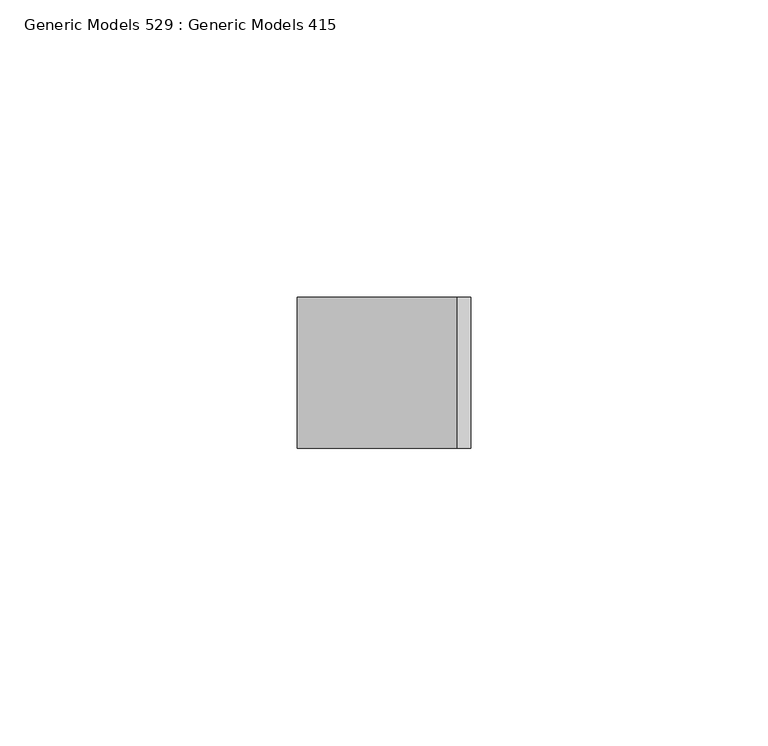
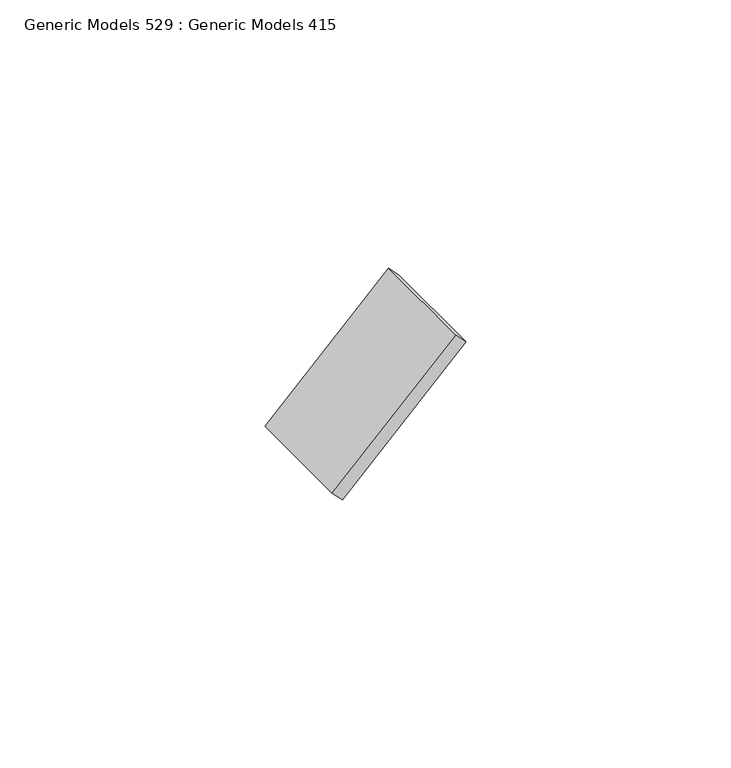
"""IFC4 building model written with IfcOpenShell, lengths in millimetres: proxy geometry, Generic Models 529 : Generic Models 415."""

from ifc_helpers import new_model, si_unit, frame, origin, place, context, project, spatial, polyline, outline, extrude, source, transform, mapped, element, save


def generic_models_529_generic_models_415_c3eaaae7(model_context):
    return source(origin(), model_context, "Body", "SweptSolid", [
        extrude(outline(polyline([(0.0, -3.175), (0.0, 0.0), (25.4, 0.0), (25.4, -3.175), (0.0, -3.175)])), frame((7848.0411784, 4501.3863946, 125384.8849742), z_axis=(0.7071067811867181, 0.0, 0.707106781186377), x_axis=(0.0, -1.0, 0.0)), (0.0, 0.0, 1.0), 38.1),
    ])


if __name__ == "__main__":
    model = new_model("IFC4")
    model_context = context("Model", 3, world=origin())
    ifc_project = project(units=[si_unit("LENGTHUNIT", "METRE", prefix="MILLI")], contexts=[model_context])
    site = spatial("IfcSite", under=ifc_project)
    building = spatial("IfcBuilding", under=site)
    placement = place(None, origin())
    generic_models_529_generic_models_415_shape = generic_models_529_generic_models_415_c3eaaae7(model_context)
    element("IfcBuildingElementProxy", 1, Name="Generic Models 529 : Generic Models 415", ObjectType="Generic Models 529 : Generic Models 415", at=placement, inside=building, context=model_context, shape_type="MappedRepresentation", body=[
        mapped(generic_models_529_generic_models_415_shape, transform((0.0, 0.0, 0.0), x_axis=(1.0, 0.0, 0.0), y_axis=(0.0, 1.0, 0.0), z_axis=(0.0, 0.0, 1.0))),
    ])
    save(model, "model.ifc")

# Revit data of these elements
# Element 1 (IfcBuildingElementProxy, "Generic Models 529 : Generic Models 415")
#   Materials on its faces: "_WELDED STEEL TABS FOR LOUVER ATTACHMENT"
# Materials
#   "_WELDED STEEL TABS FOR LOUVER ATTACHMENT": class "Metal", colour RGB 199 199 199, transparency 0, Description = "Structural steel 50ksi", Cost = 0
